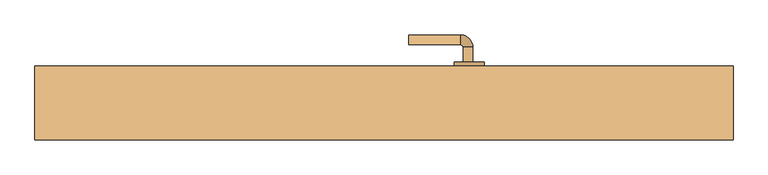
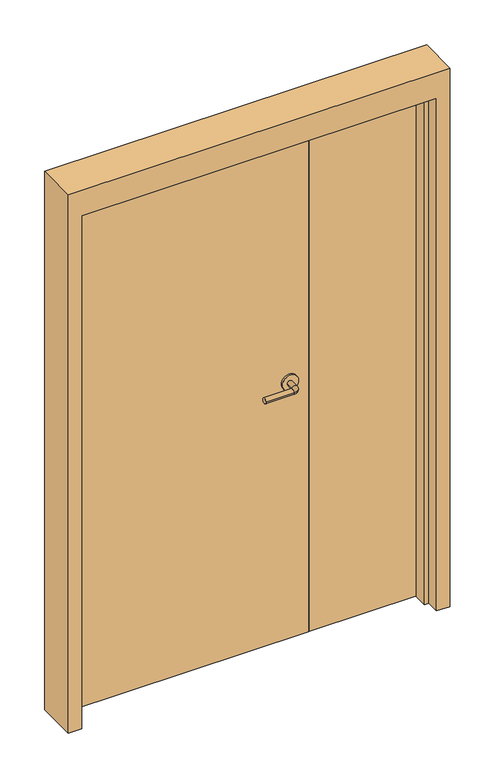
"""IFC4 building model written with IfcOpenShell, lengths in millimetres: door geometry, Дверь-Маятниковая-С полотнами разной ширины-Щитовая : 1410 x 2100 мм."""

from ifc_helpers import new_model, si_unit, point, frame, frame_2d, origin, origin_with_axes, place, context, project, spatial, polyline, circle_curve, ellipse_curve, trimmed, segment, composite_curve, outline, extrude, faceted_brep, source, transform, mapped, element, save
from ifc_brep_helpers import plane_surface, cylinder_surface, revolved_surface, advanced_brep


def door_198ad6e6(model_context):
    return source(origin(), model_context, "Body", "SolidModel", [
        advanced_brep(
        [(179.59375, 143.35, 1000.0), (159.59375, 143.35, 1000.0), (179.59375, 113.35, 1000.0), (159.59375, 113.35, 1000.0), (154.59375, 108.35, 1000.0), (154.59375, 88.35, 1000.0), (49.59375, 88.35, 1000.0), (49.59375, 108.35, 1000.0)],
        [
            (0, 1, circle_curve(frame((169.59375, 143.35, 1000.0), z_axis=(0.0, 1.0, 0.0), x_axis=(-1.0, 0.0, 0.0)), 10.0)),
            (1, 0, circle_curve(frame((169.59375, 143.35, 1000.0), z_axis=(0.0, 1.0, 0.0), x_axis=(-1.0, 0.0, 0.0)), 10.0)),
            (0, 2),
            (2, 3, circle_curve(frame((169.59375, 113.35, 1000.0), z_axis=(0.0, 1.0, 0.0), x_axis=(-1.0, 0.0, 0.0)), 10.0)),
            (3, 1),
            (3, 2, circle_curve(frame((169.59375, 113.35, 1000.0), z_axis=(0.0, 1.0, 0.0), x_axis=(-1.0, 0.0, 0.0)), 10.0)),
            (4, 3, circle_curve(frame((154.59375, 113.35, 1000.0), z_axis=(0.0, 0.0, 1.0), x_axis=(1.0, 0.0, 0.0)), 5.0)),
            (2, 5, circle_curve(frame((154.59375, 113.35, 1000.0), z_axis=(0.0, 0.0, -1.0), x_axis=(1.0, 0.0, 0.0)), 25.0)),
            (5, 4, circle_curve(frame((154.59375, 98.35, 1000.0), z_axis=(1.0, 0.0, 0.0), x_axis=(0.0, 1.0, 0.0)), 10.0)),
            (4, 5, circle_curve(frame((154.59375, 98.35, 1000.0), z_axis=(1.0, 0.0, 0.0), x_axis=(0.0, 1.0, 0.0)), 10.0)),
            (6, 7, circle_curve(frame((49.59375, 98.35, 1000.0), z_axis=(-1.0, 0.0, 0.0), x_axis=(0.0, 1.0, 0.0)), 10.0)),
            (7, 6, circle_curve(frame((49.59375, 98.35, 1000.0), z_axis=(-1.0, 0.0, 0.0), x_axis=(0.0, 1.0, 0.0)), 10.0)),
            (5, 6),
            (7, 4),
        ],
        [
            plane_surface(frame((169.59375, 143.35, 1000.0), z_axis=(0.0, 1.0, 0.0), x_axis=(0.0, 0.0, 1.0))),
            cylinder_surface(frame((169.59375, 143.35, 1000.0), z_axis=(0.0, 1.0, 0.0), x_axis=(-1.0, 0.0, 0.0)), 10.0),
            revolved_surface(trimmed(ellipse_curve(frame((169.59375, 113.35, 1000.0), z_axis=(0.0, 1.0, 0.0), x_axis=(-1.0, 0.0, 0.0)), 10.0, 10.0), [point((179.59375, 113.35, 1000.0))], [point((159.59375, 113.35, 1000.0))], True, "CARTESIAN"), (154.59375, 113.35, 1000.0), (0.0, 0.0, -1.0)),
            revolved_surface(trimmed(ellipse_curve(frame((169.59375, 113.35, 1000.0), z_axis=(0.0, 1.0, 0.0), x_axis=(-1.0, 0.0, 0.0)), 10.0, 10.0), [point((159.59375, 113.35, 1000.0))], [point((179.59375, 113.35, 1000.0))], True, "CARTESIAN"), (154.59375, 113.35, 1000.0), (0.0, 0.0, -1.0)),
            plane_surface(frame((49.59375, 98.35, 1000.0), z_axis=(-1.0, 0.0, 0.0), x_axis=(0.0, 0.0, 1.0))),
            cylinder_surface(frame((154.59375, 98.35, 1000.0), z_axis=(1.0, 0.0, 0.0), x_axis=(0.0, 1.0, 0.0)), 10.0),
        ],
        [
            (0, [[1, 2]]),
            (1, [[-1, 3, 4, 5]]),
            (1, [[-2, -5, 6, -3]]),
            (2, [[7, -4, 8, 9]]),
            (3, [[-8, -6, -7, 10]]),
            (4, [[11, 12]]),
            (5, [[-9, 13, -12, 14]]),
            (5, [[-10, -14, -11, -13]]),
        ],
    ),
        extrude(outline(composite_curve([segment(trimmed(circle_curve(frame_2d((1000.0, 172.09375)), 30.0), [point((1000.0, 202.09375))], [point((1000.0, 142.09375))], False, "CARTESIAN"), True, "CONTINUOUS"), segment(trimmed(circle_curve(frame_2d((1000.0, 172.09375)), 30.0), [point((1000.0, 142.09375))], [point((1000.0, 202.09375))], False, "CARTESIAN"), True, "CONTINUOUS")], self_intersect=False)), frame((0.0, 143.35, 0.0), z_axis=(0.0, 1.0, 0.0), x_axis=(0.0, 0.0, 1.0)), (0.0, 0.0, 1.0), 8.0),
        advanced_brep(
        [(179.59375, 204.35, 1000.0), (159.59375, 204.35, 1000.0), (159.59375, 234.35, 1000.0), (179.59375, 234.35, 1000.0), (154.59375, 239.35, 1000.0), (154.59375, 259.35, 1000.0), (49.59375, 259.35, 1000.0), (49.59375, 239.35, 1000.0)],
        [
            (0, 1, circle_curve(frame((169.59375, 204.35, 1000.0), z_axis=(0.0, -1.0, 0.0), x_axis=(-1.0, 0.0, 0.0)), 10.0)),
            (1, 0, circle_curve(frame((169.59375, 204.35, 1000.0), z_axis=(0.0, -1.0, 0.0), x_axis=(-1.0, 0.0, 0.0)), 10.0)),
            (1, 2),
            (2, 3, circle_curve(frame((169.59375, 234.35, 1000.0), z_axis=(0.0, -1.0, 0.0), x_axis=(-1.0, 0.0, 0.0)), 10.0)),
            (3, 0),
            (3, 2, circle_curve(frame((169.59375, 234.35, 1000.0), z_axis=(0.0, -1.0, 0.0), x_axis=(-1.0, 0.0, 0.0)), 10.0)),
            (4, 5, circle_curve(frame((154.59375, 249.35, 1000.0), z_axis=(1.0, 0.0, 0.0), x_axis=(0.0, -1.0, 0.0)), 10.0)),
            (5, 3, circle_curve(frame((154.59375, 234.35, 1000.0), z_axis=(0.0, 0.0, -1.0), x_axis=(1.0, 0.0, 0.0)), 25.0)),
            (2, 4, circle_curve(frame((154.59375, 234.35, 1000.0), z_axis=(0.0, 0.0, 1.0), x_axis=(1.0, 0.0, 0.0)), 5.0)),
            (5, 4, circle_curve(frame((154.59375, 249.35, 1000.0), z_axis=(1.0, 0.0, 0.0), x_axis=(0.0, -1.0, 0.0)), 10.0)),
            (6, 7, circle_curve(frame((49.59375, 249.35, 1000.0), z_axis=(-1.0, 0.0, 0.0), x_axis=(0.0, -1.0, 0.0)), 10.0)),
            (7, 6, circle_curve(frame((49.59375, 249.35, 1000.0), z_axis=(-1.0, 0.0, 0.0), x_axis=(0.0, -1.0, 0.0)), 10.0)),
            (4, 7),
            (6, 5),
        ],
        [
            plane_surface(frame((169.59375, 204.35, 1000.0), z_axis=(0.0, -1.0, 0.0), x_axis=(0.0, 0.0, 1.0))),
            cylinder_surface(frame((169.59375, 204.35, 1000.0), z_axis=(0.0, -1.0, 0.0), x_axis=(-1.0, 0.0, 0.0)), 10.0),
            revolved_surface(trimmed(ellipse_curve(frame((169.59375, 234.35, 1000.0), z_axis=(0.0, 1.0, 0.0), x_axis=(-1.0, 0.0, 0.0)), 10.0, 10.0), [point((179.59375, 234.35, 1000.0))], [point((159.59375, 234.35, 1000.0))], True, "CARTESIAN"), (154.59375, 234.35, 1000.0), (0.0, 0.0, -1.0)),
            revolved_surface(trimmed(ellipse_curve(frame((169.59375, 234.35, 1000.0), z_axis=(0.0, 1.0, 0.0), x_axis=(-1.0, 0.0, 0.0)), 10.0, 10.0), [point((159.59375, 234.35, 1000.0))], [point((179.59375, 234.35, 1000.0))], True, "CARTESIAN"), (154.59375, 234.35, 1000.0), (0.0, 0.0, -1.0)),
            plane_surface(frame((49.59375, 249.35, 1000.0), z_axis=(-1.0, 0.0, 0.0), x_axis=(0.0, 0.0, 1.0))),
            cylinder_surface(frame((154.59375, 249.35, 1000.0), z_axis=(1.0, 0.0, 0.0), x_axis=(0.0, -1.0, 0.0)), 10.0),
        ],
        [
            (0, [[1, 2]]),
            (1, [[3, 4, 5, -2]]),
            (1, [[-5, 6, -3, -1]]),
            (2, [[7, 8, -4, 9]]),
            (3, [[10, -9, -6, -8]]),
            (4, [[11, 12]]),
            (5, [[13, -11, 14, -7]]),
            (5, [[-14, -12, -13, -10]]),
        ],
    ),
        extrude(outline(composite_curve([segment(trimmed(circle_curve(frame_2d((1000.0, 172.09375)), 30.0), [point((1000.0, 202.09375))], [point((1000.0, 142.09375))], False, "CARTESIAN"), True, "CONTINUOUS"), segment(trimmed(circle_curve(frame_2d((1000.0, 172.09375)), 30.0), [point((1000.0, 142.09375))], [point((1000.0, 202.09375))], False, "CARTESIAN"), True, "CONTINUOUS")], self_intersect=False)), frame((0.0, 196.35, 0.0), z_axis=(0.0, 1.0, 0.0), x_axis=(0.0, 0.0, 1.0)), (0.0, 0.0, 1.0), 8.0),
        extrude(outline(polyline([(655.0, 151.35), (246.6, 151.35), (246.6, 196.35), (655.0, 196.35), (655.0, 151.35)])), origin_with_axes(), (0.0, 0.0, 1.0), 2000.0),
        faceted_brep([(655.0, 146.5875, 0.0), (655.0, 196.35, 0.0), (705.0, 196.35, 0.0), (705.0, 46.35, 0.0), (655.0, 46.35, 0.0), (655.0, 95.5625, 0.0), (639.125, 95.5625, 0.0), (639.125, 146.5875, 0.0), (655.0, 146.5875, 2000.0), (655.0, 196.35, 2000.0), (-655.0, 196.35, 2000.0), (-655.0, 196.35, 0.0), (-705.0, 196.35, 0.0), (-705.0, 196.35, 2100.0), (705.0, 196.35, 2100.0), (705.0, 46.35, 2100.0), (-705.0, 46.35, 2100.0), (-705.0, 46.35, 0.0), (-655.0, 46.35, 0.0), (-655.0, 46.35, 2000.0), (655.0, 46.35, 2000.0), (655.0, 95.5625, 2000.0), (-655.0, 95.5625, 2000.0), (-655.0, 95.5625, 0.0), (-639.125, 95.5625, 0.0), (-639.125, 95.5625, 1984.125), (639.125, 95.5625, 1984.125), (639.125, 146.5875, 1984.125), (-639.125, 146.5875, 1984.125), (-639.125, 146.5875, 0.0), (-655.0, 146.5875, 0.0), (-655.0, 146.5875, 2000.0)], [[[0, 1, 2, 3, 4, 5, 6, 7]], [[1, 0, 8, 9]], [[2, 1, 9, 10, 11, 12, 13, 14]], [[3, 2, 14, 15]], [[4, 3, 15, 16, 17, 18, 19, 20]], [[5, 4, 20, 21]], [[6, 5, 21, 22, 23, 24, 25, 26]], [[7, 6, 26, 27]], [[0, 7, 27, 28, 29, 30, 31, 8]], [[9, 8, 31, 10]], [[20, 19, 22, 21]], [[26, 25, 28, 27]], [[12, 11, 30, 29, 24, 23, 18, 17]], [[11, 10, 31, 30]], [[13, 12, 17, 16]], [[19, 18, 23, 22]], [[25, 24, 29, 28]], [[15, 14, 13, 16]]]),
        extrude(outline(polyline([(243.4, 151.35), (-655.0, 151.35), (-655.0, 196.35), (243.4, 196.35), (243.4, 151.35)])), origin_with_axes(), (0.0, 0.0, 1.0), 2000.0),
    ])


if __name__ == "__main__":
    model = new_model("IFC4")
    model_context = context("Model", 3, world=origin())
    ifc_project = project(units=[si_unit("LENGTHUNIT", "METRE", prefix="MILLI")], contexts=[model_context])
    site = spatial("IfcSite", under=ifc_project)
    building = spatial("IfcBuilding", under=site)
    placement = place(None, origin())
    door_shape = door_198ad6e6(model_context)
    element("IfcDoor", 1, ObjectType="Дверь-Маятниковая-С полотнами разной ширины-Щитовая : 1410 x 2100 мм", at=placement, inside=building, context=model_context, shape_type="MappedRepresentation", body=[
        mapped(door_shape, transform((0.0, 0.0, 0.0), x_axis=(1.0, 0.0, 0.0), y_axis=(0.0, 1.0, 0.0), z_axis=(0.0, 0.0, 1.0))),
    ])
    save(model, "model.ifc")

# Revit data of these elements
# Type "Дверь-Маятниковая-С полотнами разной ширины-Щитовая : 1410 x 2100 мм"
#   Type Mark = "155"
#   Assembly Code = "C1020300"
#   Analytic Construction = "Деревянный"
#   Ширина большой панели = 900 mm
#   W = 410 mm
#   Thickness = 45 mm
#   Thermal Resistance (R) = 0.455703 (m²·K)/W
#   Угол поворота [instance default] = 90°
#   Высота планки = 1000 mm
#   Rough Width [instance default] = 1410 mm
#   Rough Height [instance default] = 2100 mm
#   Высота проема в кирпичном каркасе [instance default] = 100 mm
#   Ширина проема в кирпичном каркасе [instance default] = 100 mm
#   Расчет вставки [instance default] = 105 mm
#   Кирпичная вставка [instance default] = 25 mm
#   Height = 2000 mm
#   Width = 1310 mm
#   Heat Transfer Coefficient (U) = 2.19465 W/(m²·K)
#   Глубина кирпичного каркаса = 150 mm
#   Кирпичный каркас [instance default] = yes
#   Каркас стены сухой кладки [instance default] = no
#   Материал панели = Древесина - Береза
#   Материал каркаса = Металл - Окрашенный - Серый 2
#   Материал дверной ручки = Алюминий
#   Visual Light Transmittance = 0
#   Solar Heat Gain Coefficient = 0
#   Wall Closure = (empty or 0)
#   Function = (empty or 0)
# Element 1 (IfcDoor, "Дверь-Маятниковая-С полотнами разной ширины-Щитовая : 1410 x 2100 мм")
#   Расчет вставки = 80 mm
#   Кирпичная вставка = 0 mm
#   Materials on its faces: "Алюминий", "Металл - Окрашенный - Серый 2", "Древесина - Береза"
# Materials
#   "Древесина - Береза": class "Древесина", colour RGB 166 116 52, transparency 0, Cost = 0
#   "Металл - Окрашенный - Серый 2": class "Краска", colour RGB 104 104 104, transparency 0, Cost = 0
#   "Алюминий": class "Металл", colour RGB 247 247 247, transparency 0
